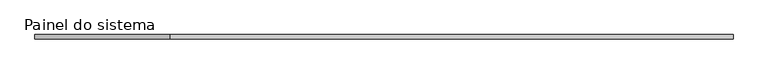
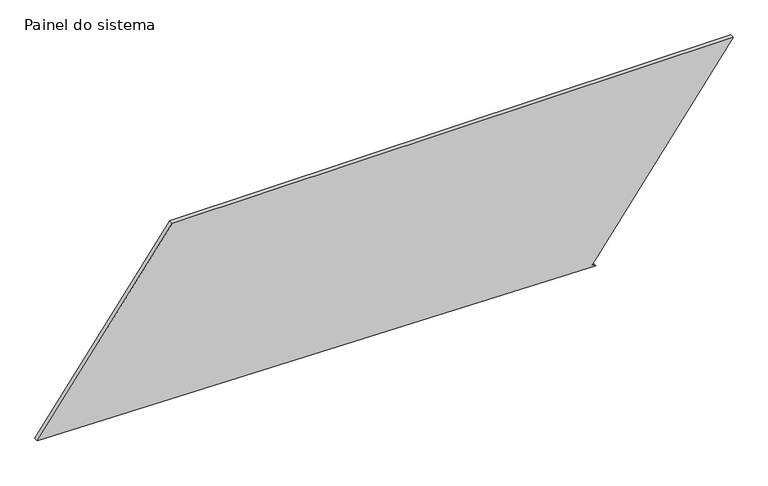
"""IFC4 building model written with IfcOpenShell, lengths in millimetres: plate geometry, Painel do sistema : Envidraçado."""

import ifcopenshell
import ifcopenshell.guid

model = None  # the IFC model being written
_history = None  # IfcOwnerHistory: only IFC2X3 demands one
_inside = {}  # id of a spatial element -> (the spatial element, [elements in it])
_under = {}  # id of a project, library or spatial element -> (it, [spatial elements below it])
_declared = {}  # id of a project -> (the project, [libraries it declares])
_typed = {}  # id of a type object -> (the type object, [elements of that type])
_made_of = {}  # id of a material, layer set ... -> (it, [elements and type objects made of it])


def new_model(schema):
    """Start an empty IFC model of exactly this schema.

    Asked for "IFC4X3", IfcOpenShell would pick the latest addendum, in which some entities
    have other attributes; the version numbers below select the first issue.
    IFC2X3 requires an IfcOwnerHistory on every rooted entity: one is made here for all.
    """
    global model, _history
    if schema == "IFC4X3":
        model = ifcopenshell.file(schema_version=(4, 3, 0, 0))
    else:
        model = ifcopenshell.file(schema=schema)
    _inside.clear()
    _under.clear()
    _declared.clear()
    _typed.clear()
    _made_of.clear()
    _history = None
    if model.schema == "IFC2X3":
        org = make("IfcOrganization", Name="unknown")
        user = make(
            "IfcPersonAndOrganization",
            ThePerson=make("IfcPerson", FamilyName="unknown"),
            TheOrganization=org,
        )
        app = make(
            "IfcApplication",
            ApplicationDeveloper=org,
            Version="unknown",
            ApplicationFullName="unknown",
            ApplicationIdentifier="unknown",
        )
        _history = make(
            "IfcOwnerHistory",
            OwningUser=user,
            OwningApplication=app,
            ChangeAction="ADDED",
            CreationDate=0,
        )
    return model


def make(cls, **values):
    """One entity of the class cls with the attributes given. An attribute that is None is left unset."""
    return model.create_entity(
        cls, **{name: value for name, value in values.items() if value is not None}
    )


def rooted(cls, **values):
    """An entity with a GlobalId (a new one), such as an element, a storey or a relation."""
    return make(cls, GlobalId=ifcopenshell.guid.new(), OwnerHistory=_history, **values)


def si_unit(unit_type, name, prefix=None):
    """IfcSIUnit, for example si_unit("LENGTHUNIT", "METRE", prefix="MILLI")."""
    return make("IfcSIUnit", UnitType=unit_type, Prefix=prefix, Name=name)


def assignment(units):
    """IfcUnitAssignment: the units of a project."""
    return None if units is None else make("IfcUnitAssignment", Units=units)


def point(xyz):
    """IfcCartesianPoint."""
    return None if xyz is None else make("IfcCartesianPoint", Coordinates=xyz)


def direction(xyz):
    """IfcDirection."""
    return None if xyz is None else make("IfcDirection", DirectionRatios=xyz)


def frame(location, z_axis=None, x_axis=None):
    """IfcAxis2Placement3D, a coordinate frame: its origin and axes. An axis left out is left unset."""
    return make(
        "IfcAxis2Placement3D",
        Location=point(location),
        Axis=direction(z_axis),
        RefDirection=direction(x_axis),
    )


def origin():
    """The frame at (0, 0, 0) with its axes left unset."""
    return frame((0.0, 0.0, 0.0))


def place(relative_to, where):
    """IfcLocalPlacement: puts the frame where relative to a parent placement (None: the world)."""
    return make(
        "IfcLocalPlacement", PlacementRelTo=relative_to, RelativePlacement=where
    )


def context(
    kind, dimensions, precision=None, world=None, true_north=None, identifier=None
):
    """IfcGeometricRepresentationContext, for example the 3D "Model" context."""
    return make(
        "IfcGeometricRepresentationContext",
        ContextIdentifier=identifier,
        ContextType=kind,
        CoordinateSpaceDimension=dimensions,
        Precision=precision,
        WorldCoordinateSystem=world,
        TrueNorth=true_north,
    )


def project(units=None, contexts=None):
    """IfcProject with its units and contexts."""
    return rooted(
        "IfcProject",
        Name="project",
        RepresentationContexts=contexts,
        UnitsInContext=assignment(units),
    )


def spatial(cls, under=None, at=None, **own):
    """A site, building, storey or space (cls), placed at a placement, below another one or the project."""
    s = rooted(cls, ObjectPlacement=at, **own)
    if under is not None:
        _under.setdefault(under.id(), (under, []))[1].append(s)
    return s


def polyline(points):
    """IfcPolyline through the points."""
    return make("IfcPolyline", Points=[point(p) for p in points])


def outline(outer, holes=None, kind="AREA"):
    """IfcArbitraryClosedProfileDef: a profile drawn as a closed curve; with holes, ...WithVoids."""
    if holes is None:
        return make("IfcArbitraryClosedProfileDef", ProfileType=kind, OuterCurve=outer)
    return make(
        "IfcArbitraryProfileDefWithVoids",
        ProfileType=kind,
        OuterCurve=outer,
        InnerCurves=holes,
    )


def extrude(swept, where, along, depth):
    """IfcExtrudedAreaSolid: the profile swept, set in the frame where, extruded along a direction by depth."""
    return make(
        "IfcExtrudedAreaSolid",
        SweptArea=swept,
        Position=where,
        ExtrudedDirection=direction(along),
        Depth=depth,
    )


def shape(context_of_items, identifier, shape_type, items):
    """IfcShapeRepresentation: the items that make up one representation, for example the "Body"."""
    return make(
        "IfcShapeRepresentation",
        ContextOfItems=context_of_items,
        RepresentationIdentifier=identifier,
        RepresentationType=shape_type,
        Items=items,
    )


def source(mapping_origin, context_of_items, identifier, shape_type, items):
    """IfcRepresentationMap: a shape defined once, which mapped items show again and again."""
    return make(
        "IfcRepresentationMap",
        MappingOrigin=mapping_origin,
        MappedRepresentation=shape(context_of_items, identifier, shape_type, items),
    )


def transform(
    local_origin,
    x_axis=None,
    y_axis=None,
    z_axis=None,
    scale=None,
    scale2=None,
    scale3=None,
    uniform=True,
):
    """IfcCartesianTransformationOperator3D, or its non-uniform kind. x_axis, y_axis, z_axis: its Axis1, 2, 3."""
    if uniform:
        return make(
            "IfcCartesianTransformationOperator3D",
            Axis1=direction(x_axis),
            Axis2=direction(y_axis),
            LocalOrigin=point(local_origin),
            Scale=scale,
            Axis3=direction(z_axis),
        )
    return make(
        "IfcCartesianTransformationOperator3DnonUniform",
        Axis1=direction(x_axis),
        Axis2=direction(y_axis),
        LocalOrigin=point(local_origin),
        Scale=scale,
        Axis3=direction(z_axis),
        Scale2=scale2,
        Scale3=scale3,
    )


def mapped(mapping_source, mapping_target):
    """IfcMappedItem: shows the shape of a source again, moved by a transform."""
    return make(
        "IfcMappedItem", MappingSource=mapping_source, MappingTarget=mapping_target
    )


def made_of(thing, what):
    """Note that an element or type object is made of a material, layer set ...; save() writes the relation."""
    if what is not None:
        _made_of.setdefault(what.id(), (what, []))[1].append(thing)
    return thing


def element(
    cls,
    number,
    at=None,
    inside=None,
    cuts=None,
    type_object=None,
    material=None,
    context=None,
    identifier="Body",
    shape_type=None,
    held_by="IfcProductDefinitionShape",
    body=None,
    shapes=None,
    **own,
):
    """One element of the class cls, such as IfcWall. Its Tag is "e" and its number.

    at: its placement. inside: the storey or other place that contains it. cuts: it is an
    opening in that element (IfcRelVoidsElement). A single representation is given by context,
    identifier, shape_type and body (its items); several are given by shapes. held_by: the class
    of the entity that holds the representations. save() writes the other relations.
    """
    e = rooted(cls, Tag="e%d" % number, ObjectPlacement=at, **own)
    if body is not None:
        shapes = [shape(context, identifier, shape_type, body)]
    if shapes is not None:
        e.Representation = make(held_by, Representations=shapes)
    if inside is not None:
        _inside.setdefault(inside.id(), (inside, []))[1].append(e)
    if cuts is not None:
        rooted(
            "IfcRelVoidsElement", RelatingBuildingElement=cuts, RelatedOpeningElement=e
        )
    if type_object is not None:
        _typed.setdefault(type_object.id(), (type_object, []))[1].append(e)
    return made_of(e, material)


def aggregate(whole, parts):
    """IfcRelAggregates: a whole, such as a stair, and the parts it consists of."""
    return rooted("IfcRelAggregates", RelatingObject=whole, RelatedObjects=parts)


def save(model, path):
    """Write the relations noted so far, then the file.

    IfcRelAggregates (storeys below a building ...), IfcRelContainedInSpatialStructure (elements
    in a storey), IfcRelDefinesByType, IfcRelAssociatesMaterial and IfcRelDeclares: one each for
    every whole, place, type object, material and project.
    """
    for whole, parts in _under.values():
        aggregate(whole, parts)
    for where, things in _inside.values():
        rooted(
            "IfcRelContainedInSpatialStructure",
            RelatedElements=things,
            RelatingStructure=where,
        )
    for kind, things in _typed.values():
        rooted("IfcRelDefinesByType", RelatedObjects=things, RelatingType=kind)
    for what, things in _made_of.values():
        rooted("IfcRelAssociatesMaterial", RelatedObjects=things, RelatingMaterial=what)
    for by, libraries in _declared.values():
        rooted("IfcRelDeclares", RelatingContext=by, RelatedDefinitions=libraries)
    model.write(path)


def painel_do_sistema_7744fe01(model_context):
    return source(origin(), model_context, "Body", "SweptSolid", [
        extrude(outline(polyline([(0.0, 1188.8313723), (14.8374505, 1168.7104861), (1092.663607, 1963.5160447), (1092.663607, -1201.8874602), (59.8283417, -1963.5160447), (0.0, 1188.8313723)])), frame((0.0, 24.5, 0.0), z_axis=(0.0, 1.0, 0.0), x_axis=(0.0, 0.0, 1.0)), (0.0, 0.0, 1.0), 25.0),
    ])


if __name__ == "__main__":
    model = new_model("IFC4")
    model_context = context("Model", 3, world=origin())
    ifc_project = project(units=[si_unit("LENGTHUNIT", "METRE", prefix="MILLI")], contexts=[model_context])
    site = spatial("IfcSite", under=ifc_project)
    building = spatial("IfcBuilding", under=site)
    placement = place(None, origin())
    painel_do_sistema_shape = painel_do_sistema_7744fe01(model_context)
    element("IfcPlate", 1, ObjectType="Painel do sistema : Envidraçado", at=placement, inside=building, context=model_context, shape_type="MappedRepresentation", body=[
        mapped(painel_do_sistema_shape, transform((0.0, 0.0, 0.0), x_axis=(1.0, 0.0, 0.0), y_axis=(0.0, 1.0, 0.0), z_axis=(0.0, 0.0, 1.0))),
    ])
    save(model, "model.ifc")

# Revit data of these elements
# Type "Painel do sistema : Envidraçado"
#   Construction Type Id = "GSP4R"
#   Analytic Construction = "Vidraça única Pilkington 1/8 pol"
#   Visual Light Transmittance = 0.9
#   Solar Heat Gain Coefficient = 0.86
#   Heat Transfer Coefficient (U) = 6.7069 W/(m²·K)
# Element 1 (IfcPlate, "Painel do sistema : Envidraçado")
#   Materials on its faces: "Vidro"
# Materials
#   "Vidro": class "Vidro", colour RGB 0 128 192, transparency 0.9, Description = "Vidro de sílica", Cost = 0
